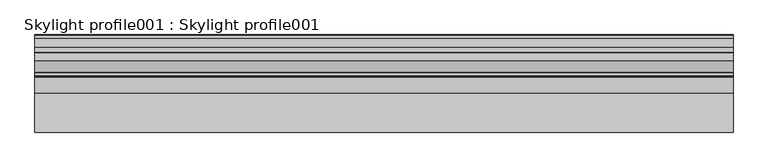
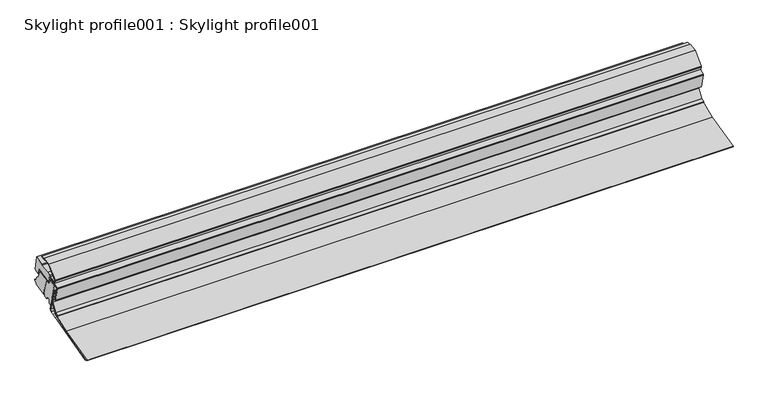
"""IFC4 building model written with IfcOpenShell, lengths in millimetres: proxy geometry, Skylight profile001 : Skylight profile001."""

from ifc_helpers import new_model, si_unit, frame, origin, place, context, project, spatial, polyline, outline, extrude, source, transform, mapped, element, save


def skylight_profile001_skylight_profile001_3bfa3745(model_context):
    return source(origin(), model_context, "Body", "SweptSolid", [
        extrude(outline(polyline([(9529.3576505, 43647.6711623), (9417.7977738, 43620.5095675), (9417.3246528, 43622.452801), (9528.7568972, 43649.5833211), (9589.2155607, 43673.0327827), (9589.9387855, 43671.1681256), (9529.3576505, 43647.6711623)])), frame((3694.2883192, 0.0, 0.0), z_axis=(1.0, 0.0, 0.0), x_axis=(0.0, 1.0, 0.0)), (0.0, 0.0, 1.0), 2000.0),
        extrude(outline(polyline([(9603.9639584, 43700.5054479), (9587.8330156, 43674.086724), (9575.8891887, 43669.7862167), (9575.211648, 43671.6679549), (9586.4929892, 43675.7299269), (9601.8204462, 43700.8327284), (9592.5767442, 43737.7822152), (9594.516951, 43738.2675993), (9603.9639584, 43700.5054479)])), frame((3694.2883192, 0.0, 0.0), z_axis=(1.0, 0.0, 0.0), x_axis=(0.0, 1.0, 0.0)), (0.0, 0.0, 1.0), 2000.0),
        extrude(outline(polyline([(9613.8776248, 43671.3606947), (9609.4651943, 43664.0246653), (9425.7655204, 43617.9331447), (9425.2787935, 43619.8730151), (9608.1771465, 43665.7634787), (9611.7375143, 43671.6828836), (9594.4616464, 43741.4763112), (9596.4030551, 43741.9568653), (9613.8776248, 43671.3606947)])), frame((3694.2883192, 0.0, 0.0), z_axis=(1.0, 0.0, 0.0), x_axis=(0.0, 1.0, 0.0)), (0.0, 0.0, 1.0), 2000.0),
        extrude(outline(polyline([(9603.3035248, 43768.2111378), (9579.627891, 43759.3071543), (9579.0362673, 43758.1814822), (9589.836091, 43715.0117709), (9587.8958843, 43714.5263868), (9576.9108524, 43758.436423), (9578.2115618, 43760.91126), (9602.7068653, 43770.1235067), (9608.5450173, 43771.5840449), (9609.0304014, 43769.6438381), (9603.3035248, 43768.2111378)])), frame((3694.2883192, 0.0, 0.0), z_axis=(1.0, 0.0, 0.0), x_axis=(0.0, 1.0, 0.0)), (0.0, 0.0, 1.0), 2000.0),
        extrude(outline(polyline([(9645.0672166, 43810.7448228), (9644.4548349, 43815.0599326), (9622.4771809, 43810.6457496), (9590.2981236, 43779.3768871), (9590.1710895, 43777.9698492), (9591.8291283, 43771.3424198), (9593.3340619, 43770.4398277), (9615.6674335, 43776.0235989), (9616.1525398, 43774.0833227), (9593.0156633, 43768.2986598), (9590.0899861, 43770.0533507), (9588.1487662, 43777.812697), (9588.3728619, 43780.2947946), (9621.5058432, 43812.4905991), (9646.1374154, 43817.437818), (9646.7372911, 43813.2108305), (9659.5391678, 43816.3334987), (9660.0131173, 43814.3904671), (9645.0672166, 43810.7448228)])), frame((3694.2883192, 0.0, 0.0), z_axis=(1.0, 0.0, 0.0), x_axis=(0.0, 1.0, 0.0)), (0.0, 0.0, 1.0), 2000.0),
        extrude(outline(polyline([(9672.3114652, 43765.1903372), (9670.4553908, 43766.1962448), (9623.0463352, 43754.3358586), (9616.8613336, 43779.0589225), (9629.0935073, 43782.1190615), (9660.4891757, 43785.4440875), (9659.6120656, 43789.7827906), (9687.9870414, 43796.8813958), (9694.3377259, 43751.9926947), (9693.1491947, 43750.2275809), (9678.7227226, 43746.6184913), (9672.3114652, 43765.1903372)])), frame((3694.2883192, 0.0, 0.0), z_axis=(1.0, 0.0, 0.0), x_axis=(0.0, 1.0, 0.0)), (0.0, 0.0, 1.0), 2000.0),
        extrude(outline(polyline([(9689.475878, 43706.8037471), (9650.7520097, 43697.1161457), (9647.279193, 43699.1990742), (9646.7464033, 43701.3287736), (9648.5983378, 43701.7920745), (9637.0159368, 43748.0899511), (9635.1640023, 43747.6266502), (9634.6775407, 43749.5711641), (9636.7604692, 43753.0439808), (9667.7800466, 43760.8041895), (9671.2528633, 43758.7212609), (9675.7442733, 43740.9813035), (9688.175753, 43730.1920963), (9690.7976108, 43719.9252266), (9691.9552163, 43719.2309171), (9696.9023539, 43718.4778099), (9696.759928, 43715.1551973), (9691.0387865, 43707.8204765), (9689.475878, 43706.8037471)])), frame((3694.2883192, 0.0, 0.0), z_axis=(1.0, 0.0, 0.0), x_axis=(0.0, 1.0, 0.0)), (0.0, 0.0, 1.0), 2000.0),
        extrude(outline(polyline([(9632.0226951, 43701.7775274), (9619.9854477, 43698.7661533), (9618.7959335, 43686.1699212), (9612.5567495, 43684.6090563), (9604.7966767, 43715.6280904), (9603.8707473, 43715.3964494), (9592.8673693, 43759.3799855), (9614.8125618, 43764.8700434), (9617.1493935, 43755.5291179), (9623.2321013, 43750.2499166), (9632.9176503, 43752.6729632), (9634.2380448, 43747.3950021), (9637.0159368, 43748.0899511), (9648.5983378, 43701.7920745), (9643.0425537, 43700.4021767), (9644.7335843, 43693.6426868), (9634.6869888, 43691.1293168), (9632.0226951, 43701.7775274)])), frame((3694.2883192, 0.0, 0.0), z_axis=(1.0, 0.0, 0.0), x_axis=(0.0, 1.0, 0.0)), (0.0, 0.0, 1.0), 2000.0),
    ])


if __name__ == "__main__":
    model = new_model("IFC4")
    model_context = context("Model", 3, world=origin())
    ifc_project = project(units=[si_unit("LENGTHUNIT", "METRE", prefix="MILLI")], contexts=[model_context])
    site = spatial("IfcSite", under=ifc_project)
    building = spatial("IfcBuilding", under=site)
    placement = place(None, origin())
    skylight_profile001_skylight_profile001_shape = skylight_profile001_skylight_profile001_3bfa3745(model_context)
    element("IfcBuildingElementProxy", 1, Name="Skylight profile001 : Skylight profile001", ObjectType="Skylight profile001 : Skylight profile001", at=placement, inside=building, context=model_context, shape_type="MappedRepresentation", body=[
        mapped(skylight_profile001_skylight_profile001_shape, transform((0.0, 0.0, 0.0), x_axis=(1.0, 0.0, 0.0), y_axis=(0.0, 1.0, 0.0), z_axis=(0.0, 0.0, 1.0))),
    ])
    save(model, "model.ifc")

# Revit data of these elements
# Type "Skylight profile001 : Skylight profile001"
#   NameOverride = "Skylight profile001"
# Element 1 (IfcBuildingElementProxy, "Skylight profile001 : Skylight profile001")
#   Materials on its faces: "IfcSurfaceStyle #732"
# Materials
#   "IfcSurfaceStyle #732": class "Unassigned", colour RGB 169 181 186, transparency 0
